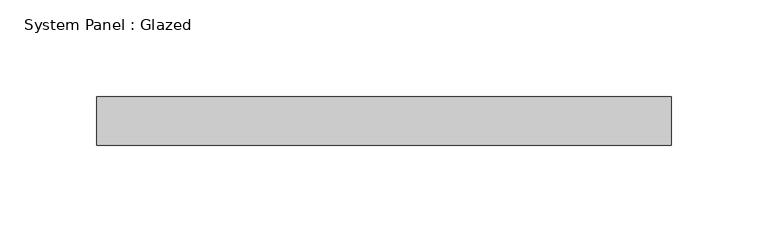
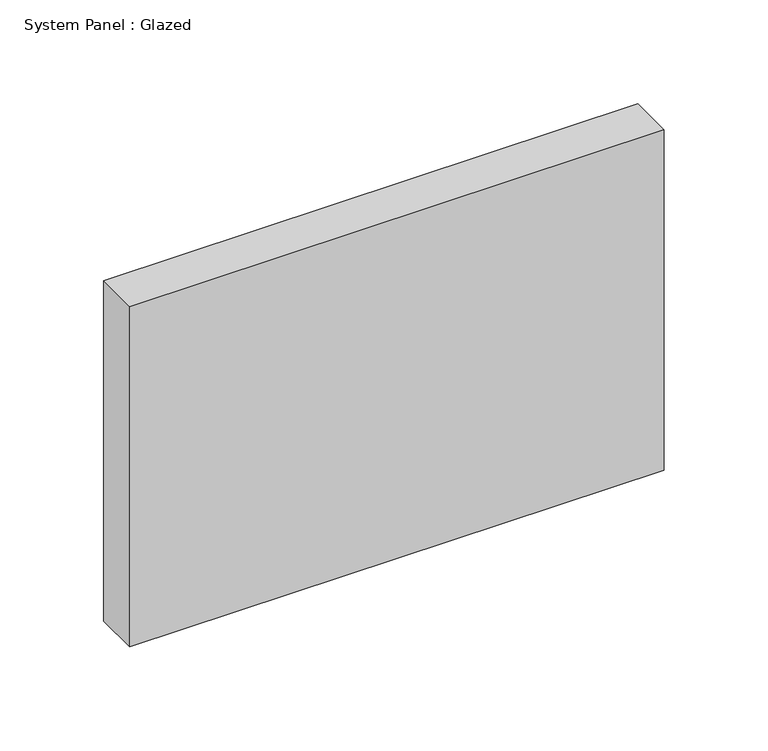
"""IFC4 building model written with IfcOpenShell, lengths in millimetres: plate geometry, System Panel : Glazed."""

from ifc_helpers import new_model, si_unit, origin, origin_with_axes, place, context, project, spatial, polyline, outline, extrude, source, transform, mapped, element, save


def system_panel_glazed_2fc8f5ca(model_context):
    return source(origin(), model_context, "Body", "SweptSolid", [
        extrude(outline(polyline([(148.4832393, 24.5), (-148.4832393, 24.5), (-148.4832393, 49.5), (148.4832393, 49.5), (148.4832393, 24.5)])), origin_with_axes(), (0.0, 0.0, 1.0), 200.0),
    ])


if __name__ == "__main__":
    model = new_model("IFC4")
    model_context = context("Model", 3, world=origin())
    ifc_project = project(units=[si_unit("LENGTHUNIT", "METRE", prefix="MILLI")], contexts=[model_context])
    site = spatial("IfcSite", under=ifc_project)
    building = spatial("IfcBuilding", under=site)
    placement = place(None, origin())
    system_panel_glazed_shape = system_panel_glazed_2fc8f5ca(model_context)
    element("IfcPlate", 1, ObjectType="System Panel : Glazed", at=placement, inside=building, context=model_context, shape_type="MappedRepresentation", body=[
        mapped(system_panel_glazed_shape, transform((0.0, 0.0, 0.0), x_axis=(1.0, 0.0, 0.0), y_axis=(0.0, 1.0, 0.0), z_axis=(0.0, 0.0, 1.0))),
    ])
    save(model, "model.ifc")

# Revit data of these elements
# Element 1 (IfcPlate, "System Panel : Glazed")
#   Materials on its faces: "Glass"
# Materials
#   "Glass": class "Glass", colour RGB 218 227 224, transparency 0.85, Description = "Soda Lime Glass", Cost = 0
